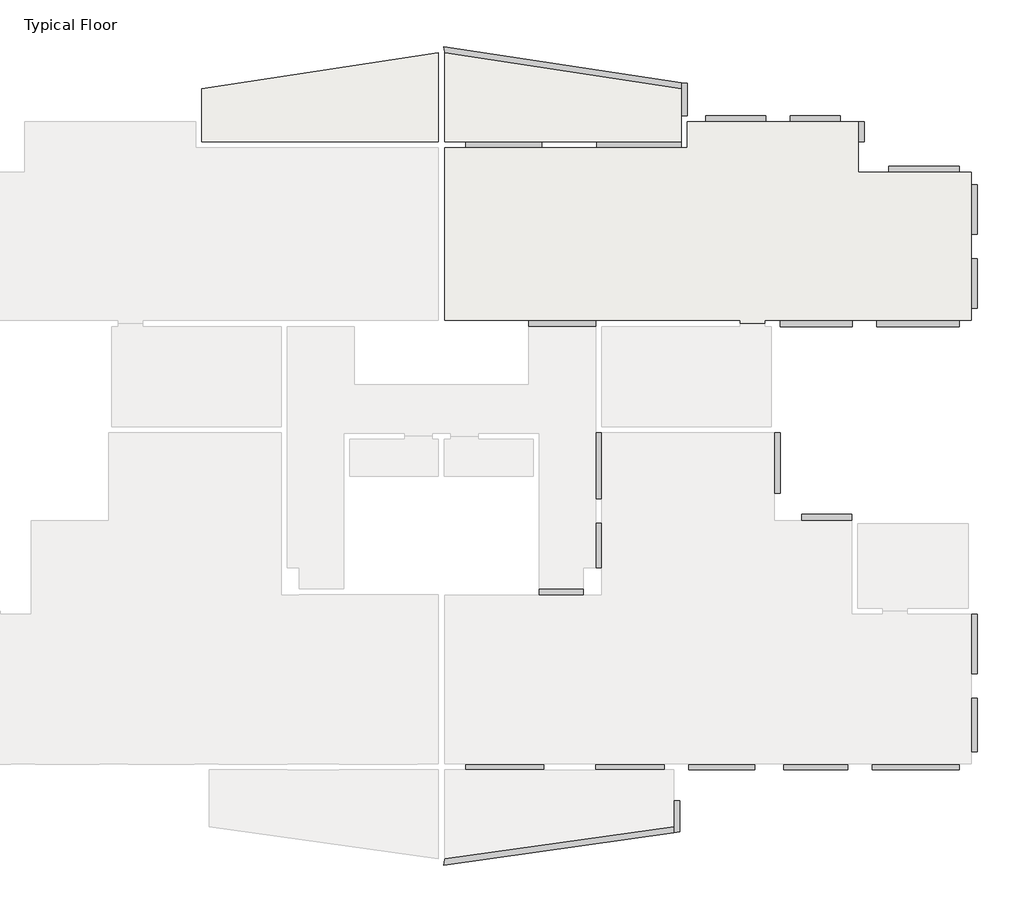
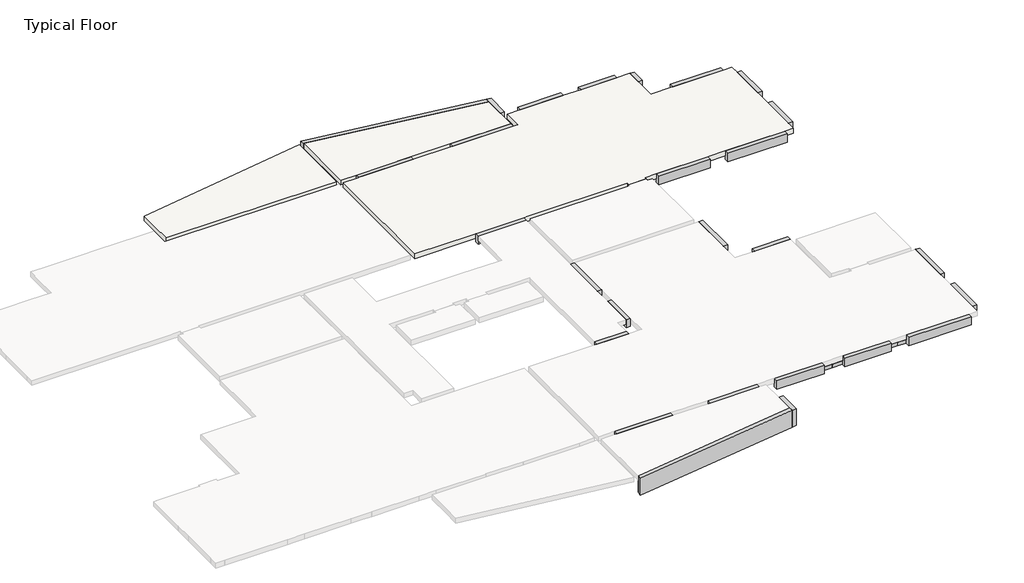
# One storey, part 2 of 2: 27 beams, 3 slabs.
"""IFC4 building model written with IfcOpenShell, lengths in millimetres."""

from ifc_helpers import new_model, si_unit, frame, origin, place, context, project, spatial, polyline, outline, extrude, faceted_brep, element, save

model = new_model("IFC4")

# Units and contexts
model_context = context("Model", 3, world=origin())
ifc_project = project(units=[si_unit("LENGTHUNIT", "METRE", prefix="MILLI")], contexts=[model_context])

# Site, building, storey
site = spatial("IfcSite", under=ifc_project)
building = spatial("IfcBuilding", under=site)
storey = spatial("IfcBuildingStorey", under=building, Name="Typical Floor", Elevation=3120.0)

# Beams
placement = place(None, origin())
element("IfcBeam", 1, ObjectType="Concrete Rectengular Beam : 20/40", at=placement, inside=storey, context=model_context, shape_type="Brep", body=[
    faceted_brep([(733.5348901, -13204.5252202, 3120.0), (733.5348901, -13009.5252202, 3120.0), (-1816.392751, -13009.5252202, 3120.0), (-1816.392751, -13204.5252202, 3120.0), (1583.607249, -13004.5252202, 2890.0), (1583.607249, -13004.5252202, 2720.0), (-1816.392751, -13004.5252202, 2720.0), (-1816.392751, -13004.5252202, 2890.0), (1583.607249, -13005.5744243, 2720.0), (733.5348901, -13005.5744243, 2720.0), (733.5348901, -13204.5252202, 2720.0), (-1816.392751, -13204.5252202, 2720.0), (733.5348901, -13204.5252202, 2890.0), (1583.607249, -13005.5744243, 2890.0), (733.5348901, -13005.5744243, 2890.0), (733.5348901, -13009.5252202, 2890.0), (-1816.392751, -13009.5252202, 2890.0)], [[[0, 1, 2, 3]], [[4, 5, 6, 7]], [[5, 8, 9, 10, 11, 6]], [[10, 12, 0, 3, 11]], [[9, 8, 13, 14]], [[10, 9, 14, 15, 1, 0, 12]], [[14, 13, 4, 7, 16, 15]], [[1, 15, 16, 2]], [[8, 5, 4, 13]], [[3, 2, 16, 7, 6, 11]]]),
])
element("IfcBeam", 2, ObjectType="Concrete Rectengular Beam : 20/40", at=placement, inside=storey, context=model_context, shape_type="Brep", body=[
    faceted_brep([(2433.5348901, -13009.5252202, 3120.0), (2433.5348901, -13204.5252202, 3120.0), (4683.408262, -13204.5252202, 3120.0), (4683.408262, -13009.5252202, 3120.0), (1583.607249, -13004.5252202, 2720.0), (1583.607249, -13004.5252202, 2890.0), (4683.408262, -13004.5252202, 2890.0), (4683.408262, -13004.5252202, 2720.0), (1583.607249, -13005.5744243, 2720.0), (4683.408262, -13204.5252202, 2720.0), (2433.5348901, -13204.5252202, 2720.0), (2433.5348901, -13005.5744243, 2720.0), (2433.5348901, -13204.5252202, 2890.0), (2433.5348901, -13005.5744243, 2890.0), (1583.607249, -13005.5744243, 2890.0), (2433.5348901, -13009.5252202, 2890.0), (4683.408262, -13009.5252202, 2890.0)], [[[0, 1, 2, 3]], [[4, 5, 6, 7]], [[8, 4, 7, 9, 10, 11]], [[1, 12, 10, 9, 2]], [[8, 11, 13, 14]], [[11, 10, 12, 1, 0, 15, 13]], [[14, 13, 15, 16, 6, 5]], [[15, 0, 3, 16]], [[3, 2, 9, 7, 6, 16]], [[4, 8, 14, 5]]]),
])
element("IfcBeam", 3, ObjectType="Concrete Rectengular Beam : 20/40", at=placement, inside=storey, context=model_context, shape_type="Brep", body=[
    faceted_brep([(7633.7700565, -13204.5252202, 3120.0), (7633.7700565, -13009.5252202, 3120.0), (5483.408262, -13009.5252202, 3120.0), (5483.408262, -13204.5252202, 3120.0), (8108.7700565, -13004.5252202, 2890.0), (8108.7700565, -13004.5252202, 2720.0), (5483.408262, -13004.5252202, 2720.0), (5483.408262, -13004.5252202, 2890.0), (8108.7700565, -13005.8747137, 2720.0), (7633.7700565, -13005.8747137, 2720.0), (7633.7700565, -13204.5252202, 2720.0), (5483.408262, -13204.5252202, 2720.0), (8108.7700565, -13005.8747137, 2890.0), (7633.7700565, -13005.8747137, 2890.0), (7633.7700565, -13009.5252202, 2890.0), (5483.408262, -13009.5252202, 2890.0)], [[[0, 1, 2, 3]], [[4, 5, 6, 7]], [[5, 8, 9, 10, 11, 6]], [[10, 0, 3, 11]], [[9, 8, 12, 13]], [[10, 9, 13, 14, 1, 0]], [[13, 12, 4, 7, 15, 14]], [[1, 14, 15, 2]], [[3, 2, 15, 7, 6, 11]], [[8, 5, 4, 12]]]),
])
element("IfcBeam", 4, ObjectType="Concrete Rectengular Beam : 20/40", at=placement, inside=storey, context=model_context, shape_type="Brep", body=[
    faceted_brep([(8583.7700565, -13204.5252202, 3120.0), (10683.6434285, -13204.5252202, 3120.0), (10683.6434285, -13009.5252202, 3120.0), (8583.7700565, -13009.5252202, 3120.0), (11083.6434285, -13004.5252202, 2720.0), (8108.7700565, -13004.5252202, 2720.0), (8108.7700565, -13004.5252202, 2890.0), (11083.6434285, -13004.5252202, 2890.0), (11083.6434285, -13005.8747137, 2720.0), (10683.6434285, -13005.8747137, 2720.0), (10683.6434285, -13204.5252202, 2720.0), (8583.7700565, -13204.5252202, 2720.0), (8583.7700565, -13005.8747137, 2720.0), (8108.7700565, -13005.8747137, 2720.0), (11083.6434285, -13005.8747137, 2890.0), (10683.6434285, -13005.8747137, 2890.0), (10683.6434285, -13009.5252202, 2890.0), (8583.7700565, -13005.8747137, 2890.0), (8108.7700565, -13005.8747137, 2890.0), (8583.7700565, -13009.5252202, 2890.0)], [[[0, 1, 2, 3]], [[4, 5, 6, 7]], [[5, 4, 8, 9, 10, 11, 12, 13]], [[10, 1, 0, 11]], [[9, 8, 14, 15]], [[10, 9, 15, 16, 2, 1]], [[13, 12, 17, 18]], [[12, 11, 0, 3, 19, 17]], [[19, 16, 15, 14, 7, 6, 18, 17]], [[16, 19, 3, 2]], [[8, 4, 7, 14]], [[5, 13, 18, 6]]]),
])
element("IfcBeam", 5, ObjectType="Concrete Rectengular Beam : 20/40", at=placement, inside=storey, context=model_context, shape_type="Brep", body=[
    faceted_brep([(11483.6434285, -13204.5252202, 3120.0), (14331.4545717, -13204.5252202, 3120.0), (14331.4545717, -13009.5252202, 3120.0), (11483.6434285, -13009.5252202, 3120.0), (14331.4545717, -13004.5252202, 2720.0), (11083.6434285, -13004.5252202, 2720.0), (11083.6434285, -13004.5252202, 2890.0), (14331.4545717, -13004.5252202, 2890.0), (14331.4545717, -13204.5252202, 2720.0), (11483.6434285, -13204.5252202, 2720.0), (11483.6434285, -13005.8747137, 2720.0), (11083.6434285, -13005.8747137, 2720.0), (14331.4545717, -13009.5252202, 2890.0), (11483.6434285, -13005.8747137, 2890.0), (11083.6434285, -13005.8747137, 2890.0), (11483.6434285, -13009.5252202, 2890.0)], [[[0, 1, 2, 3]], [[4, 5, 6, 7]], [[5, 4, 8, 9, 10, 11]], [[8, 1, 0, 9]], [[8, 4, 7, 12, 2, 1]], [[11, 10, 13, 14]], [[10, 9, 0, 3, 15, 13]], [[15, 12, 7, 6, 14, 13]], [[12, 15, 3, 2]], [[5, 11, 14, 6]]]),
])
element("IfcBeam", 6, ObjectType="Concrete Rectengular Beam : 20/40", at=placement, inside=storey, context=model_context, shape_type="SweptSolid", body=[
    extrude(outline(polyline([(14731.4545717, -12604.5252202), (14731.4545717, -10455.1764503), (14732.5037758, -10455.1764503), (14732.5037758, -10855.1764503), (14931.4545717, -10855.1764503), (14931.4545717, -12604.5252202), (14731.4545717, -12604.5252202)])), frame((0.0, 0.0, 2720.0), z_axis=(0.0, 0.0, 1.0), x_axis=(1.0, 0.0, 0.0)), (0.0, 0.0, 1.0), 400.0),
])
element("IfcBeam", 7, ObjectType="Concrete Rectengular Beam : 20/40", at=placement, inside=storey, context=model_context, shape_type="Brep", body=[
    faceted_brep([(14731.4545717, -10455.1764503, 3120.0), (14732.5037758, -10455.1764503, 3120.0), (14732.5037758, -10055.1764503, 3120.0), (14931.4545717, -10055.1764503, 3120.0), (14931.4545717, -8105.8819496, 3120.0), (14731.4545717, -8105.8819496, 3120.0), (14731.4545717, -10455.1764503, 2720.0), (14731.4545717, -8105.8819496, 2890.0), (14731.4545717, -8105.8819496, 2720.0), (14732.5037758, -10455.1764503, 2720.0), (14931.4545717, -8105.8819496, 2720.0), (14931.4545717, -10055.1764503, 2720.0), (14732.5037758, -10055.1764503, 2720.0)], [[[0, 1, 2, 3, 4, 5]], [[6, 0, 5, 7, 8]], [[9, 6, 8, 10, 11, 12]], [[3, 11, 10, 4]], [[12, 2, 1, 9]], [[2, 12, 11, 3]], [[5, 4, 10, 8, 7]], [[0, 6, 9, 1]]]),
])
element("IfcBeam", 8, ObjectType="Concrete Rectengular Beam : 20/40", at=placement, inside=storey, context=model_context, shape_type="Brep", body=[
    faceted_brep([(10812.4856861, -4836.9600972, 3120.0), (10812.4856861, -5036.9600972, 3120.0), (10812.4856861, -5036.9600972, 2890.0), (10812.4856861, -5036.9600972, 2720.0), (10812.4856861, -4836.9600972, 2720.0), (9182.4856861, -4836.9600972, 3120.0), (9182.4856861, -5036.9600972, 3120.0), (9182.4856861, -4836.9600972, 2720.0), (9182.4856861, -5036.9600972, 2720.0), (9182.4856861, -5036.9600972, 2890.0)], [[[0, 1, 2, 3, 4]], [[1, 0, 5, 6]], [[0, 4, 7, 5]], [[4, 3, 8, 7]], [[1, 6, 9, 8, 3, 2]], [[6, 5, 7, 8, 9]]]),
])
element("IfcBeam", 9, ObjectType="Concrete Rectengular Beam : 20/40", at=placement, inside=storey, context=model_context, shape_type="Brep", body=[
    faceted_brep([(8282.4856861, -4136.9600972, 3120.0), (8482.4856861, -4136.9600972, 3120.0), (8482.4856861, -2169.1055386, 3120.0), (8282.4856861, -2169.1055386, 3120.0), (8282.4856861, -2169.1055386, 2890.0), (8282.4856861, -2169.1055386, 2720.0), (8282.4856861, -4136.9600972, 2720.0), (8282.4856861, -4136.9600972, 2890.0), (8482.4856861, -4136.9600972, 2720.0), (8482.4856861, -2169.1055386, 2720.0)], [[[0, 1, 2, 3]], [[0, 3, 4, 5, 6, 7]], [[8, 6, 5, 9]], [[1, 8, 9, 2]], [[1, 0, 7, 6, 8]], [[3, 2, 9, 5, 4]]]),
])
element("IfcBeam", 10, ObjectType="Concrete Rectengular Beam : 20/40", at=placement, inside=storey, context=model_context, shape_type="Brep", body=[
    faceted_brep([(583.5168004, -7475.6540191, 3120.0), (583.5168004, -7475.1655965, 3120.0), (583.5168004, -7475.1655965, 2720.0), (583.5168004, -7475.6540191, 2720.0), (583.5168004, -7475.6540191, 2890.0), (2033.5168004, -7475.6540191, 3120.0), (2033.5168004, -7275.6540191, 3120.0), (583.7157874, -7275.6540191, 3120.0), (583.7157874, -7475.1655965, 3120.0), (2033.5168004, -7475.6540191, 2720.0), (2033.5168004, -7475.6540191, 2890.0), (583.7157874, -7475.1655965, 2720.0), (583.7157874, -7275.6540191, 2720.0), (2033.5168004, -7275.6540191, 2720.0), (2033.5168004, -7275.6540191, 2890.0), (583.7157874, -7275.6540191, 2890.0)], [[[0, 1, 2, 3, 4]], [[0, 5, 6, 7, 8, 1]], [[5, 0, 4, 3, 9, 10]], [[9, 3, 2, 11, 12, 13]], [[6, 14, 13, 12, 15, 7]], [[6, 5, 10, 9, 13, 14]], [[2, 1, 8, 11]], [[11, 8, 7, 15, 12]]]),
])
element("IfcBeam", 11, ObjectType="Concrete Rectengular Beam : 20/40", at=placement, inside=storey, context=model_context, shape_type="Brep", body=[
    faceted_brep([(2433.5348901, -6575.6540191, 3120.0), (2633.5348901, -6575.6540191, 3120.0), (2633.5348901, -5121.583831, 3120.0), (2433.5348901, -5121.583831, 3120.0), (2433.5348901, -6575.6540191, 2720.0), (2433.5348901, -6575.6540191, 2890.0), (2433.5348901, -5121.583831, 2720.0), (2633.5348901, -6575.6540191, 2720.0), (2633.5348901, -5121.583831, 2720.0), (2633.5348901, -6575.6540191, 2890.0), (2633.5348901, -5121.583831, 2890.0)], [[[0, 1, 2, 3]], [[4, 5, 0, 3, 6]], [[7, 4, 6, 8]], [[2, 1, 9, 7, 8, 10]], [[3, 2, 10, 8, 6]], [[1, 0, 5, 4, 7, 9]]]),
])
element("IfcBeam", 12, ObjectType="Concrete Rectengular Beam : 20/40", at=placement, inside=storey, context=model_context, shape_type="Brep", body=[
    faceted_brep([(2433.5348901, -4321.583831, 3120.0), (2633.5348901, -4321.583831, 3120.0), (2633.5348901, -2169.1055386, 3120.0), (2433.5348901, -2169.1055386, 3120.0), (2433.5348901, -4321.583831, 2720.0), (2433.5348901, -2169.1055386, 2720.0), (2633.5348901, -4321.583831, 2720.0), (2633.5348901, -2169.1055386, 2720.0), (2633.5348901, -4321.583831, 2890.0), (2633.5348901, -2169.1055386, 2890.0)], [[[0, 1, 2, 3]], [[4, 0, 3, 5]], [[6, 4, 5, 7]], [[2, 1, 8, 6, 7, 9]], [[1, 0, 4, 6, 8]], [[3, 2, 9, 7, 5]]]),
])
element("IfcBeam", 13, ObjectType="Concrete Rectengular Beam : 20/40", at=placement, inside=storey, context=model_context, shape_type="Brep", body=[
    faceted_brep([(2433.5348901, 1313.6006842, 3120.0), (2433.5348901, 1513.6006842, 3120.0), (247.1926325, 1513.6006842, 3120.0), (247.1926325, 1313.6006842, 3120.0), (2433.5348901, 1313.6006842, 2720.0), (2433.5348901, 1313.6006842, 2890.0), (247.1926325, 1313.6006842, 2890.0), (247.1926325, 1313.6006842, 2720.0), (2433.5348901, 1513.6006842, 2720.0), (247.1926325, 1513.6006842, 2720.0), (2433.5348901, 1513.6006842, 2890.0), (247.1926325, 1513.6006842, 2890.0)], [[[0, 1, 2, 3]], [[4, 5, 0, 3, 6, 7]], [[8, 4, 7, 9]], [[2, 1, 10, 8, 9, 11]], [[1, 0, 5, 4, 8, 10]], [[3, 2, 11, 9, 7, 6]]]),
])
element("IfcBeam", 14, ObjectType="Concrete Rectengular Beam : 20/40", at=placement, inside=storey, context=model_context, shape_type="Brep", body=[
    faceted_brep([(11629.7179581, 1514.1252863, 3120.0), (11629.7179581, 1314.1252863, 3120.0), (14331.4545717, 1314.1252863, 3120.0), (14331.4545717, 1514.1252863, 3120.0), (11629.7179581, 1314.1252863, 2720.0), (14331.4545717, 1314.1252863, 2720.0), (11629.7179581, 1514.1252863, 2720.0), (14331.4545717, 1514.1252863, 2720.0), (11629.7179581, 1514.1252863, 2890.0)], [[[0, 1, 2, 3]], [[1, 4, 5, 2]], [[4, 6, 7, 5]], [[6, 8, 0, 3, 7]], [[1, 0, 8, 6, 4]], [[3, 2, 5, 7]]]),
])
element("IfcBeam", 15, ObjectType="Concrete Rectengular Beam : 20/40", at=placement, inside=storey, context=model_context, shape_type="Brep", body=[
    faceted_brep([(10829.7179581, 1314.1252863, 3120.0), (10829.7179581, 1514.1252863, 3120.0), (8482.4856861, 1514.1252863, 3120.0), (8482.4856861, 1314.1252863, 3120.0), (10829.7179581, 1314.1252863, 2720.0), (8482.4856861, 1314.1252863, 2720.0), (10829.7179581, 1514.1252863, 2720.0), (8482.4856861, 1514.1252863, 2720.0), (10829.7179581, 1514.1252863, 2890.0), (8482.4856861, 1514.1252863, 2890.0)], [[[0, 1, 2, 3]], [[4, 0, 3, 5]], [[6, 4, 5, 7]], [[2, 1, 8, 6, 7, 9]], [[1, 0, 4, 6, 8]], [[3, 2, 9, 7, 5]]]),
])
element("IfcBeam", 16, ObjectType="Concrete Rectengular Beam : 20/40", at=placement, inside=storey, context=model_context, shape_type="Brep", body=[
    faceted_brep([(14931.4545717, 3539.1252863, 3120.0), (14736.4545717, 3539.1252863, 3120.0), (14736.4545717, 1914.1252863, 3120.0), (14931.4545717, 1914.1252863, 3120.0), (14731.4545717, 3934.6498883, 2890.0), (14731.4545717, 3934.6498883, 2720.0), (14731.4545717, 1914.1252863, 2720.0), (14731.4545717, 1914.1252863, 2890.0), (14732.5037758, 3934.6498883, 2720.0), (14732.5037758, 3539.1252863, 2720.0), (14931.4545717, 3539.1252863, 2720.0), (14931.4545717, 1914.1252863, 2720.0), (14732.5037758, 3934.6498883, 2890.0), (14732.5037758, 3539.1252863, 2890.0), (14736.4545717, 3539.1252863, 2890.0), (14736.4545717, 1914.1252863, 2890.0)], [[[0, 1, 2, 3]], [[4, 5, 6, 7]], [[5, 8, 9, 10, 11, 6]], [[10, 0, 3, 11]], [[9, 8, 12, 13]], [[10, 9, 13, 14, 1, 0]], [[13, 12, 4, 7, 15, 14]], [[1, 14, 15, 2]], [[3, 2, 15, 7, 6, 11]], [[8, 5, 4, 12]]]),
])
element("IfcBeam", 17, ObjectType="Concrete Rectengular Beam : 20/40", at=placement, inside=storey, context=model_context, shape_type="Brep", body=[
    faceted_brep([(14931.4545717, 4339.1252863, 3120.0), (14931.4545717, 5963.5645048, 3120.0), (14736.4545717, 5963.5645048, 3120.0), (14736.4545717, 4339.1252863, 3120.0), (14731.4545717, 5963.5645048, 2720.0), (14731.4545717, 3934.6498883, 2720.0), (14731.4545717, 3934.6498883, 2890.0), (14731.4545717, 5963.5645048, 2890.0), (14931.4545717, 5963.5645048, 2720.0), (14931.4545717, 4339.1252863, 2720.0), (14732.5037758, 4339.1252863, 2720.0), (14732.5037758, 3934.6498883, 2720.0), (14736.4545717, 5963.5645048, 2890.0), (14736.4545717, 4339.1252863, 2890.0), (14732.5037758, 4339.1252863, 2890.0), (14732.5037758, 3934.6498883, 2890.0)], [[[0, 1, 2, 3]], [[4, 5, 6, 7]], [[5, 4, 8, 9, 10, 11]], [[8, 1, 0, 9]], [[8, 4, 7, 12, 2, 1]], [[10, 9, 0, 3, 13, 14]], [[11, 10, 14, 15]], [[13, 12, 7, 6, 15, 14]], [[12, 13, 3, 2]], [[5, 11, 15, 6]]]),
])
element("IfcBeam", 18, ObjectType="Concrete Rectengular Beam : 20/40", at=placement, inside=storey, context=model_context, shape_type="Brep", body=[
    faceted_brep([(14331.4545717, 6363.5645048, 3120.0), (14331.4545717, 6563.5645048, 3120.0), (12031.8163662, 6563.5645048, 3120.0), (12031.8163662, 6363.5645048, 3120.0), (12031.8163662, 6363.5645048, 2890.0), (12031.8163662, 6363.5645048, 2720.0), (14331.4545717, 6363.5645048, 2720.0), (14331.4545717, 6363.5645048, 2890.0), (14331.4545717, 6563.5645048, 2720.0), (12031.8163662, 6563.5645048, 2720.0)], [[[0, 1, 2, 3]], [[0, 3, 4, 5, 6, 7]], [[8, 6, 5, 9]], [[1, 8, 9, 2]], [[1, 0, 7, 6, 8]], [[3, 2, 9, 5, 4]]]),
])
element("IfcBeam", 19, ObjectType="Concrete Rectengular Beam : 20/40", at=placement, inside=storey, context=model_context, shape_type="Brep", body=[
    faceted_brep([(11031.8163662, 7363.5645048, 3120.0), (11231.8163662, 7363.5645048, 3120.0), (11231.8163662, 8012.3163138, 3120.0), (11031.8163662, 8012.3163138, 3120.0), (11031.8163662, 8012.3163138, 2890.0), (11031.8163662, 8012.3163138, 2720.0), (11031.8163662, 7363.5645048, 2720.0), (11031.8163662, 7363.5645048, 2890.0), (11231.8163662, 7363.5645048, 2720.0), (11231.8163662, 8012.3163138, 2720.0)], [[[0, 1, 2, 3]], [[0, 3, 4, 5, 6, 7]], [[8, 6, 5, 9]], [[1, 8, 9, 2]], [[1, 0, 7, 6, 8]], [[3, 2, 9, 5, 4]]]),
])
element("IfcBeam", 20, ObjectType="Concrete Rectengular Beam : 20/40", at=placement, inside=storey, context=model_context, shape_type="SweptSolid", body=[
    extrude(outline(polyline([(10431.7801868, 8212.3163138), (10431.7801868, 8012.3163138), (8806.3098539, 8012.3163138), (8806.3098539, 8212.3163138), (10431.7801868, 8212.3163138)])), frame((0.0, 0.0, 2720.0), z_axis=(0.0, 0.0, 1.0), x_axis=(1.0, 0.0, 0.0)), (0.0, 0.0, 1.0), 400.0),
])
element("IfcBeam", 21, ObjectType="Concrete Rectengular Beam : 20/40", at=placement, inside=storey, context=model_context, shape_type="SweptSolid", body=[
    extrude(outline(polyline([(6033.6615182, 8012.3163138), (6033.6615182, 8212.3163138), (8006.3098539, 8212.3163138), (8006.3098539, 8012.3163138), (6033.6615182, 8012.3163138)])), frame((0.0, 0.0, 2720.0), z_axis=(0.0, 0.0, 1.0), x_axis=(1.0, 0.0, 0.0)), (0.0, 0.0, 1.0), 400.0),
])
element("IfcBeam", 22, ObjectType="Concrete Rectengular Beam : 20/40", at=placement, inside=storey, context=model_context, shape_type="Brep", body=[
    faceted_brep([(5233.6615182, 7363.6006842, 3120.0), (2472.6086962, 7363.6006842, 3120.0), (2472.6086962, 7168.6006842, 3120.0), (5233.6615182, 7168.6006842, 3120.0), (5233.6615182, 7363.6006842, 2890.0), (5233.6615182, 7363.6006842, 2720.0), (2472.6086962, 7363.6006842, 2720.0), (5233.6615182, 7163.6006842, 2720.0), (2472.6086962, 7163.6006842, 2720.0), (5233.6615182, 7163.6006842, 2890.0), (2472.6086962, 7163.6006842, 2890.0), (5233.6615182, 7168.6006842, 2890.0), (2472.6086962, 7168.6006842, 2890.0)], [[[0, 1, 2, 3]], [[0, 4, 5, 6, 1]], [[5, 7, 8, 6]], [[8, 7, 9, 10]], [[5, 4, 0, 3, 11, 9, 7]], [[1, 6, 8, 10, 12, 2]], [[11, 12, 10, 9]], [[12, 11, 3, 2]]]),
])
element("IfcBeam", 23, ObjectType="Concrete Rectengular Beam : 20/40", at=placement, inside=storey, context=model_context, shape_type="SweptSolid", body=[
    extrude(outline(polyline([(7363.6006842, 2720.0), (7163.6006842, 2720.0), (7163.6006842, 2890.0), (7168.6006842, 2890.0), (7168.6006842, 3120.0), (7363.6006842, 3120.0), (7363.6006842, 2720.0)])), frame((-1816.392751, 0.0, 0.0), z_axis=(1.0, 0.0, 0.0), x_axis=(0.0, 1.0, 0.0)), (0.0, 0.0, 1.0), 2489.0014472),
])
element("IfcBeam", 24, ObjectType="Concrete Rectengular Beam : 20/80", at=placement, inside=storey, context=model_context, shape_type="Brep", body=[
    faceted_brep([(5433.6615182, 9273.3163139, 3120.0), (5233.6615182, 9303.5953834, 3120.0), (5233.6615182, 9101.3163136, 3120.0), (5233.6615182, 8212.3163138, 3120.0), (5433.6615182, 8212.3163138, 3120.0), (5233.6615182, 9303.5953834, 2320.0), (5233.6615182, 9101.3163136, 2320.0), (5233.6615182, 8212.3163138, 2320.0), (5433.6615182, 9273.3163139, 2320.0), (5433.6615182, 8212.3163138, 2320.0)], [[[0, 1, 2, 3, 4]], [[1, 5, 6, 7, 3, 2]], [[5, 8, 9, 7, 6]], [[8, 0, 4, 9]], [[4, 3, 7, 9]], [[1, 0, 8, 5]]]),
])
element("IfcBeam", 25, ObjectType="Concrete Rectengular Beam : 20/80", at=placement, inside=storey, context=model_context, shape_type="Brep", body=[
    faceted_brep([(5233.6615182, 9101.3163136, 3120.0), (5233.6615182, 9303.5953834, 3120.0), (-2543.043603, 10480.9523568, 3120.0), (-2516.392751, 10304.9175415, 3120.0), (-2516.392751, 10274.6384721, 3120.0), (5233.6615182, 9101.3163136, 2320.0), (5233.6615182, 9101.3163136, 2890.0), (-2516.392751, 10274.6384721, 2890.0), (-2516.392751, 10274.6384721, 2320.0), (5233.6615182, 9303.5953834, 2320.0), (-2516.392751, 10304.9175415, 2320.0), (-2543.043603, 10480.9523568, 2320.0)], [[[0, 1, 2, 3, 4]], [[5, 6, 0, 4, 7, 8]], [[9, 5, 8, 10, 11]], [[1, 9, 11, 2]], [[1, 0, 6, 5, 9]], [[4, 3, 10, 8, 7]], [[3, 2, 11, 10]]]),
])
element("IfcBeam", 26, ObjectType="Concrete Rectengular Beam : 20/80", at=placement, inside=storey, context=model_context, shape_type="Brep", body=[
    faceted_brep([(4983.408262, -15260.611265, 3120.0), (5183.408262, -15232.5030981, 3120.0), (5183.408262, -14204.5252202, 3120.0), (4983.408262, -14204.5252202, 3120.0), (4983.408262, -15058.6457505, 3120.0), (5183.408262, -15232.5030981, 2320.0), (5183.408262, -14204.5252202, 2320.0), (4983.408262, -15260.611265, 2320.0), (4983.408262, -15058.6457505, 2320.0), (4983.408262, -14204.5252202, 2320.0)], [[[0, 1, 2, 3, 4]], [[1, 5, 6, 2]], [[5, 7, 8, 9, 6]], [[7, 0, 4, 3, 9, 8]], [[3, 2, 6, 9]], [[1, 0, 7, 5]]]),
])
element("IfcBeam", 27, ObjectType="Concrete Rectengular Beam : 20/80", at=placement, inside=storey, context=model_context, shape_type="Brep", body=[
    faceted_brep([(4983.408262, -15260.611265, 3120.0), (4983.408262, -15058.6457505, 3120.0), (-2516.392751, -16112.674045, 3120.0), (-2516.392751, -16140.7822119, 3120.0), (-2541.3191471, -16318.142736, 3120.0), (4983.408262, -15260.611265, 2320.0), (-2541.3191471, -16318.142736, 2320.0), (4983.408262, -15058.6457505, 2320.0), (-2516.392751, -16140.7822119, 2320.0), (-2516.392751, -16112.674045, 2320.0), (4983.408262, -15058.6457505, 2890.0), (-2516.392751, -16112.674045, 2890.0)], [[[0, 1, 2, 3, 4]], [[5, 0, 4, 6]], [[7, 5, 6, 8, 9]], [[1, 10, 7, 9, 11, 2]], [[1, 0, 5, 7, 10]], [[3, 2, 11, 9, 8]], [[4, 3, 8, 6]]]),
])

# Slabs
element("IfcSlab", 28, ObjectType="23", at=placement, inside=storey, context=model_context, shape_type="Brep", body=[
    faceted_brep([(-2716.392751, 7363.6006842, 2890.0), (-10466.4470202, 7363.6006842, 2890.0), (-10466.4470202, 9101.3163136, 2890.0), (-2716.392751, 10274.6384721, 2890.0), (-10466.4470202, 7363.6006842, 3120.0), (-7705.3941982, 7363.6006842, 3120.0), (-5905.3941982, 7363.6006842, 3120.0), (-3416.392751, 7363.6006842, 3120.0), (-2716.392751, 7363.6006842, 3120.0), (-2716.392751, 10274.6384721, 3120.0), (-10466.4470202, 9101.3163136, 3120.0), (-10466.4470202, 8212.3163138, 3120.0)], [[[0, 1, 2, 3]], [[4, 5, 6, 7, 8, 9, 10, 11]], [[1, 0, 8, 7, 6, 5, 4]], [[2, 1, 4, 11, 10]], [[3, 2, 10, 9]], [[0, 3, 9, 8]]]),
])
element("IfcSlab", 29, ObjectType="23", at=placement, inside=storey, context=model_context, shape_type="Brep", body=[
    faceted_brep([(7163.9075385, 1413.6006842, 2890.0), (7163.9075385, 1513.6006842, 2890.0), (2633.5348901, 1513.6006842, 2890.0), (2433.5348901, 1513.6006842, 2890.0), (247.1926325, 1513.6006842, 2890.0), (47.1926325, 1513.6006842, 2890.0), (-2516.392751, 1513.6006842, 2890.0), (-2516.392751, 6363.6006842, 2890.0), (-2516.392751, 7163.6006842, 2890.0), (-1816.392751, 7163.6006842, 2890.0), (-1816.392751, 7168.6006842, 2890.0), (672.6086962, 7168.6006842, 2890.0), (672.6086962, 7163.6006842, 2890.0), (2472.6086962, 7163.6006842, 2890.0), (2472.6086962, 7168.6006842, 2890.0), (5233.6615182, 7168.6006842, 2890.0), (5233.6615182, 7163.6006842, 2890.0), (5233.6615182, 7162.3163138, 2890.0), (5433.6615182, 7162.3163138, 2890.0), (5433.6615182, 8012.3163138, 2890.0), (6033.6615182, 8012.3163138, 2890.0), (11031.8163662, 8012.3163138, 2890.0), (11031.8163662, 7363.5645048, 2890.0), (11031.8163662, 6363.5645048, 2890.0), (12031.8163662, 6363.5645048, 2890.0), (14331.4545717, 6363.5645048, 2890.0), (14731.4545717, 6363.5645048, 2890.0), (14731.4545717, 5963.5645048, 2890.0), (14736.4545717, 5963.5645048, 2890.0), (14736.4545717, 4339.1252863, 2890.0), (14732.5037758, 4339.1252863, 2890.0), (14732.5037758, 3934.6498883, 2890.0), (14732.5037758, 3539.1252863, 2890.0), (14736.4545717, 3539.1252863, 2890.0), (14736.4545717, 1914.1252863, 2890.0), (14731.4545717, 1914.1252863, 2890.0), (14731.4545717, 1514.1252863, 2890.0), (14331.4545717, 1514.1252863, 2890.0), (11629.7179581, 1514.1252863, 2890.0), (10829.7179581, 1514.1252863, 2890.0), (8482.4856861, 1514.1252863, 2890.0), (7963.9075385, 1514.1252863, 2890.0), (7963.9075385, 1413.6006842, 2890.0), (7962.4856861, 1413.6006842, 2890.0), (7163.9075385, 1513.6006842, 3120.0), (7163.9075385, 1413.6006842, 3120.0), (7962.4856861, 1413.6006842, 3120.0), (7963.9075385, 1413.6006842, 3120.0), (7963.9075385, 1514.1252863, 3120.0), (8482.4856861, 1514.1252863, 3120.0), (10829.7179581, 1514.1252863, 3120.0), (11629.7179581, 1514.1252863, 3120.0), (14331.4545717, 1514.1252863, 3120.0), (14731.4545717, 1514.1252863, 3120.0), (14731.4545717, 1914.1252863, 3120.0), (14736.4545717, 1914.1252863, 3120.0), (14736.4545717, 3539.1252863, 3120.0), (14732.5037758, 3539.1252863, 3120.0), (14732.5037758, 4339.1252863, 3120.0), (14736.4545717, 4339.1252863, 3120.0), (14736.4545717, 5963.5645048, 3120.0), (14731.4545717, 5963.5645048, 3120.0), (14731.4545717, 6363.5645048, 3120.0), (14331.4545717, 6363.5645048, 3120.0), (12031.8163662, 6363.5645048, 3120.0), (11031.8163662, 6363.5645048, 3120.0), (11031.8163662, 7363.5645048, 3120.0), (11031.8163662, 8012.3163138, 3120.0), (10431.7801868, 8012.3163138, 3120.0), (8806.3098539, 8012.3163138, 3120.0), (8006.3098539, 8012.3163138, 3120.0), (6033.6615182, 8012.3163138, 3120.0), (5433.6615182, 8012.3163138, 3120.0), (5433.6615182, 7162.3163138, 3120.0), (5233.6615182, 7162.3163138, 3120.0), (5233.6615182, 7168.6006842, 3120.0), (2472.6086962, 7168.6006842, 3120.0), (2472.6086962, 7163.6006842, 3120.0), (672.6086962, 7163.6006842, 3120.0), (672.6086962, 7168.6006842, 3120.0), (-1816.392751, 7168.6006842, 3120.0), (-1816.392751, 7163.6006842, 3120.0), (-2516.392751, 7163.6006842, 3120.0), (-2516.392751, 6363.6006842, 3120.0), (-2516.392751, 1513.6006842, 3120.0), (47.1926325, 1513.6006842, 3120.0), (247.1926325, 1513.6006842, 3120.0), (2433.5348901, 1513.6006842, 3120.0), (2633.5348901, 1513.6006842, 3120.0)], [[[0, 1, 2, 3, 4, 5, 6, 7, 8, 9, 10, 11, 12, 13, 14, 15, 16, 17, 18, 19, 20, 21, 22, 23, 24, 25, 26, 27, 28, 29, 30, 31, 32, 33, 34, 35, 36, 37, 38, 39, 40, 41, 42, 43]], [[44, 45, 46, 47, 48, 49, 50, 51, 52, 53, 54, 55, 56, 57, 58, 59, 60, 61, 62, 63, 64, 65, 66, 67, 68, 69, 70, 71, 72, 73, 74, 75, 76, 77, 78, 79, 80, 81, 82, 83, 84, 85, 86, 87, 88]], [[72, 19, 18, 73]], [[75, 15, 14, 76]], [[10, 80, 79, 11]], [[6, 84, 83, 82, 8, 7]], [[1, 44, 88, 87, 86, 85, 84, 6, 5, 4, 3, 2]], [[1, 0, 45, 44]], [[0, 43, 42, 47, 46, 45]], [[42, 41, 48, 47]], [[48, 41, 40, 39, 38, 37, 36, 53, 52, 51, 50, 49]], [[55, 34, 33, 56]], [[28, 60, 59, 29]], [[23, 65, 64, 63, 62, 26, 25, 24]], [[21, 67, 66, 65, 23, 22]], [[67, 21, 20, 19, 72, 71, 70, 69, 68]], [[9, 81, 80, 10]], [[81, 9, 8, 82]], [[54, 35, 34, 55]], [[35, 54, 53, 36]], [[61, 27, 26, 62]], [[27, 61, 60, 28]], [[74, 17, 16, 15, 75]], [[73, 18, 17, 74]], [[78, 12, 11, 79]], [[12, 78, 77, 13]], [[13, 77, 76, 14]], [[58, 30, 29, 59]], [[30, 58, 57, 32, 31]], [[32, 57, 56, 33]]]),
])
element("IfcSlab", 30, ObjectType="23", at=placement, inside=storey, context=model_context, shape_type="Brep", body=[
    faceted_brep([(5233.6615182, 7363.6006842, 2890.0), (-2516.392751, 7363.6006842, 2890.0), (-2516.392751, 10274.6384721, 2890.0), (5233.6615182, 9101.3163136, 2890.0), (-2516.392751, 7363.6006842, 3120.0), (-1816.392751, 7363.6006842, 3120.0), (672.6086962, 7363.6006842, 3120.0), (2472.6086962, 7363.6006842, 3120.0), (5233.6615182, 7363.6006842, 3120.0), (5233.6615182, 8212.3163138, 3120.0), (5233.6615182, 9101.3163136, 3120.0), (-2516.392751, 10274.6384721, 3120.0)], [[[0, 1, 2, 3]], [[4, 5, 6, 7, 8, 9, 10, 11]], [[1, 0, 8, 7, 6, 5, 4]], [[0, 3, 10, 9, 8]], [[3, 2, 11, 10]], [[2, 1, 4, 11]]]),
])

save(model, "model.ifc")

# Revit data of these elements
# Type "Concrete Rectengular Beam : 20/40"
#   Keynote = "09000"
#   Length [instance default] = 152.4 cm
#   b = 20 cm
#   h = 40 cm
#   Structural Material [instance default] = Concrete
#   Assembly Code = ""
# Type "Concrete Rectengular Beam : 20/80"
#   Length [instance default] = 152.4 cm
#   b = 20 cm
#   h = 80 cm
#   Structural Material [instance default] = Concrete
#   Assembly Code = ""
# Type "23"
#   Function = 0
#   Layers, outside or top first: 23 cm "Concrete" (function 1)
# Element 1 (IfcBeam, "Concrete Rectengular Beam : 20/40")
#   Comments = ""
#   Mark = "B24"
#   SOFiSTiK_AMG_Comments = ""
#   SOFiSTiK_AMG_Scheduled = yes
#   SOFiSTiK_AMG_Adjusted = yes
#   Structural Material = Concrete
#   Phase Created = New Construction
#   Materials on its faces: "Concrete"
# Element 2 (IfcBeam, "Concrete Rectengular Beam : 20/40")
#   Comments = ""
#   Mark = "B25"
#   SOFiSTiK_AMG_Comments = ""
#   SOFiSTiK_AMG_Scheduled = yes
#   SOFiSTiK_AMG_Adjusted = yes
#   Structural Material = Concrete
#   Phase Created = New Construction
#   Materials on its faces: "Concrete"
# Element 3 (IfcBeam, "Concrete Rectengular Beam : 20/40")
#   Comments = ""
#   Mark = "B26"
#   SOFiSTiK_AMG_Comments = ""
#   SOFiSTiK_AMG_Scheduled = yes
#   SOFiSTiK_AMG_Adjusted = yes
#   Structural Material = Concrete
#   Phase Created = New Construction
#   Materials on its faces: "Concrete"
# Element 4 (IfcBeam, "Concrete Rectengular Beam : 20/40")
#   Comments = ""
#   Mark = "B27"
#   SOFiSTiK_AMG_Comments = ""
#   SOFiSTiK_AMG_Scheduled = yes
#   SOFiSTiK_AMG_Adjusted = yes
#   Structural Material = Concrete
#   Phase Created = New Construction
#   Materials on its faces: "Concrete"
# Element 5 (IfcBeam, "Concrete Rectengular Beam : 20/40")
#   Comments = ""
#   Mark = "B28"
#   SOFiSTiK_AMG_Comments = ""
#   SOFiSTiK_AMG_Scheduled = yes
#   SOFiSTiK_AMG_Adjusted = yes
#   Structural Material = Concrete
#   Phase Created = New Construction
#   Materials on its faces: "Concrete"
# Element 6 (IfcBeam, "Concrete Rectengular Beam : 20/40")
#   Comments = ""
#   Mark = "B29"
#   SOFiSTiK_AMG_Comments = ""
#   SOFiSTiK_AMG_Scheduled = yes
#   SOFiSTiK_AMG_Adjusted = yes
#   Structural Material = Concrete
#   Phase Created = New Construction
#   Materials on its faces: "Concrete"
# Element 7 (IfcBeam, "Concrete Rectengular Beam : 20/40")
#   Comments = ""
#   Mark = "B30"
#   SOFiSTiK_AMG_Comments = ""
#   SOFiSTiK_AMG_Scheduled = yes
#   SOFiSTiK_AMG_Adjusted = yes
#   Structural Material = Concrete
#   Phase Created = New Construction
#   Materials on its faces: "Concrete"
# Element 8 (IfcBeam, "Concrete Rectengular Beam : 20/40")
#   Comments = ""
#   Mark = "B31"
#   SOFiSTiK_AMG_Comments = ""
#   SOFiSTiK_AMG_Scheduled = yes
#   SOFiSTiK_AMG_Adjusted = yes
#   Structural Material = Concrete
#   Phase Created = New Construction
#   Materials on its faces: "Concrete"
# Element 9 (IfcBeam, "Concrete Rectengular Beam : 20/40")
#   Comments = ""
#   Mark = "B32"
#   SOFiSTiK_AMG_Comments = ""
#   SOFiSTiK_AMG_Scheduled = yes
#   SOFiSTiK_AMG_Adjusted = yes
#   Structural Material = Concrete
#   Phase Created = New Construction
#   Materials on its faces: "Concrete"
# Element 10 (IfcBeam, "Concrete Rectengular Beam : 20/40")
#   Comments = ""
#   Mark = "B33"
#   SOFiSTiK_AMG_Comments = ""
#   SOFiSTiK_AMG_Scheduled = yes
#   SOFiSTiK_AMG_Adjusted = yes
#   Structural Material = Concrete
#   Phase Created = New Construction
#   Materials on its faces: "Concrete"
# Element 11 (IfcBeam, "Concrete Rectengular Beam : 20/40")
#   Comments = ""
#   Mark = "B34"
#   SOFiSTiK_AMG_Comments = ""
#   SOFiSTiK_AMG_Scheduled = yes
#   SOFiSTiK_AMG_Adjusted = yes
#   Structural Material = Concrete
#   Phase Created = New Construction
#   Materials on its faces: "Concrete"
# Element 12 (IfcBeam, "Concrete Rectengular Beam : 20/40")
#   Comments = ""
#   Mark = "B35"
#   SOFiSTiK_AMG_Comments = ""
#   SOFiSTiK_AMG_Scheduled = yes
#   SOFiSTiK_AMG_Adjusted = yes
#   Structural Material = Concrete
#   Phase Created = New Construction
#   Materials on its faces: "Concrete"
# Element 13 (IfcBeam, "Concrete Rectengular Beam : 20/40")
#   Comments = ""
#   Mark = "B36"
#   SOFiSTiK_AMG_Comments = ""
#   SOFiSTiK_AMG_Scheduled = yes
#   SOFiSTiK_AMG_Adjusted = yes
#   Structural Material = Concrete
#   Phase Created = New Construction
#   Materials on its faces: "Concrete"
# Element 14 (IfcBeam, "Concrete Rectengular Beam : 20/40")
#   Comments = ""
#   Mark = "B37"
#   SOFiSTiK_AMG_Comments = ""
#   SOFiSTiK_AMG_Scheduled = yes
#   SOFiSTiK_AMG_Adjusted = yes
#   Structural Material = Concrete
#   Phase Created = New Construction
#   Materials on its faces: "Concrete"
# Element 15 (IfcBeam, "Concrete Rectengular Beam : 20/40")
#   Comments = ""
#   Mark = "B38"
#   SOFiSTiK_AMG_Comments = ""
#   SOFiSTiK_AMG_Scheduled = yes
#   SOFiSTiK_AMG_Adjusted = yes
#   Structural Material = Concrete
#   Phase Created = New Construction
#   Materials on its faces: "Concrete"
# Element 16 (IfcBeam, "Concrete Rectengular Beam : 20/40")
#   Comments = ""
#   Mark = "B39"
#   SOFiSTiK_AMG_Comments = ""
#   SOFiSTiK_AMG_Scheduled = yes
#   SOFiSTiK_AMG_Adjusted = yes
#   Structural Material = Concrete
#   Phase Created = New Construction
#   Materials on its faces: "Concrete"
# Element 17 (IfcBeam, "Concrete Rectengular Beam : 20/40")
#   Comments = ""
#   Mark = "B40"
#   SOFiSTiK_AMG_Comments = ""
#   SOFiSTiK_AMG_Scheduled = yes
#   SOFiSTiK_AMG_Adjusted = yes
#   Structural Material = Concrete
#   Phase Created = New Construction
#   Materials on its faces: "Concrete"
# Element 18 (IfcBeam, "Concrete Rectengular Beam : 20/40")
#   Comments = ""
#   Mark = "B41"
#   SOFiSTiK_AMG_Comments = ""
#   SOFiSTiK_AMG_Scheduled = yes
#   SOFiSTiK_AMG_Adjusted = yes
#   Structural Material = Concrete
#   Phase Created = New Construction
#   Materials on its faces: "Concrete"
# Element 19 (IfcBeam, "Concrete Rectengular Beam : 20/40")
#   Comments = ""
#   Mark = "B42"
#   SOFiSTiK_AMG_Comments = ""
#   SOFiSTiK_AMG_Scheduled = yes
#   SOFiSTiK_AMG_Adjusted = yes
#   Structural Material = Concrete
#   Phase Created = New Construction
#   Materials on its faces: "Concrete"
# Element 20 (IfcBeam, "Concrete Rectengular Beam : 20/40")
#   Comments = ""
#   Mark = "B43"
#   SOFiSTiK_AMG_Comments = ""
#   SOFiSTiK_AMG_Scheduled = yes
#   SOFiSTiK_AMG_Adjusted = yes
#   Structural Material = Concrete
#   Phase Created = New Construction
#   Materials on its faces: "Concrete"
# Element 21 (IfcBeam, "Concrete Rectengular Beam : 20/40")
#   Comments = ""
#   Mark = "B44"
#   SOFiSTiK_AMG_Comments = ""
#   SOFiSTiK_AMG_Scheduled = yes
#   SOFiSTiK_AMG_Adjusted = yes
#   Structural Material = Concrete
#   Phase Created = New Construction
#   Materials on its faces: "Concrete"
# Element 22 (IfcBeam, "Concrete Rectengular Beam : 20/40")
#   Comments = ""
#   Mark = "B45"
#   SOFiSTiK_AMG_Comments = ""
#   SOFiSTiK_AMG_Scheduled = yes
#   SOFiSTiK_AMG_Adjusted = yes
#   Structural Material = Concrete
#   Phase Created = New Construction
#   Materials on its faces: "Concrete"
# Element 23 (IfcBeam, "Concrete Rectengular Beam : 20/40")
#   Comments = ""
#   Mark = "B46"
#   SOFiSTiK_AMG_Comments = ""
#   SOFiSTiK_AMG_Scheduled = yes
#   SOFiSTiK_AMG_Adjusted = yes
#   Structural Material = Concrete
#   Phase Created = New Construction
#   Materials on its faces: "Concrete"
# Element 24 (IfcBeam, "Concrete Rectengular Beam : 20/80")
#   Comments = ""
#   Mark = "B53"
#   SOFiSTiK_AMG_Comments = ""
#   SOFiSTiK_AMG_Scheduled = yes
#   SOFiSTiK_AMG_Adjusted = yes
#   Structural Material = Concrete
#   Phase Created = New Construction
#   Materials on its faces: "Concrete"
# Element 25 (IfcBeam, "Concrete Rectengular Beam : 20/80")
#   Comments = ""
#   Mark = "B54"
#   SOFiSTiK_AMG_Comments = ""
#   SOFiSTiK_AMG_Scheduled = yes
#   SOFiSTiK_AMG_Adjusted = yes
#   Structural Material = Concrete
#   Phase Created = New Construction
#   Materials on its faces: "Concrete"
# Element 26 (IfcBeam, "Concrete Rectengular Beam : 20/80")
#   Comments = ""
#   Mark = "B55"
#   SOFiSTiK_AMG_Comments = ""
#   SOFiSTiK_AMG_Scheduled = yes
#   SOFiSTiK_AMG_Adjusted = yes
#   Structural Material = Concrete
#   Phase Created = New Construction
#   Materials on its faces: "Concrete"
# Element 27 (IfcBeam, "Concrete Rectengular Beam : 20/80")
#   Comments = ""
#   Mark = "B56"
#   SOFiSTiK_AMG_Comments = ""
#   SOFiSTiK_AMG_Scheduled = yes
#   SOFiSTiK_AMG_Adjusted = yes
#   Structural Material = Concrete
#   Phase Created = New Construction
#   Materials on its faces: "Concrete"
# Element 28 (IfcSlab, "23")
#   Mark = "S6"
#   SOFiSTiK_AMG_Comments = ""
#   Height Offset From Level = 0 cm
#   built-in parameter 1001954 = 1
#   SOFiSTiK_AMG_Scheduled = yes
#   SOFiSTiK_AMG_Adjusted = yes
#   Phase Created = New Construction
#   Materials on its faces: "Concrete"
# Element 29 (IfcSlab, "23")
#   Mark = "S10"
#   SOFiSTiK_AMG_Comments = ""
#   built-in parameter 1001955 = 3.14159 (stored number, unit not read)
#   Height Offset From Level = 0 cm
#   built-in parameter 1001954 = 1
#   SOFiSTiK_AMG_Scheduled = yes
#   SOFiSTiK_AMG_Adjusted = yes
#   Phase Created = New Construction
#   Materials on its faces: "Concrete"
# Element 30 (IfcSlab, "23")
#   Mark = "S12"
#   SOFiSTiK_AMG_Comments = ""
#   built-in parameter 1001955 = 3.14159 (stored number, unit not read)
#   Height Offset From Level = 0 cm
#   built-in parameter 1001954 = 1
#   SOFiSTiK_AMG_Scheduled = yes
#   SOFiSTiK_AMG_Adjusted = yes
#   Phase Created = New Construction
#   Materials on its faces: "Concrete"
# Materials
#   "Concrete": class "Concrete", colour RGB 192 192 192, transparency 0, Keynote = "01000", Description = "Cast-in-place concrete", Cost = 0
